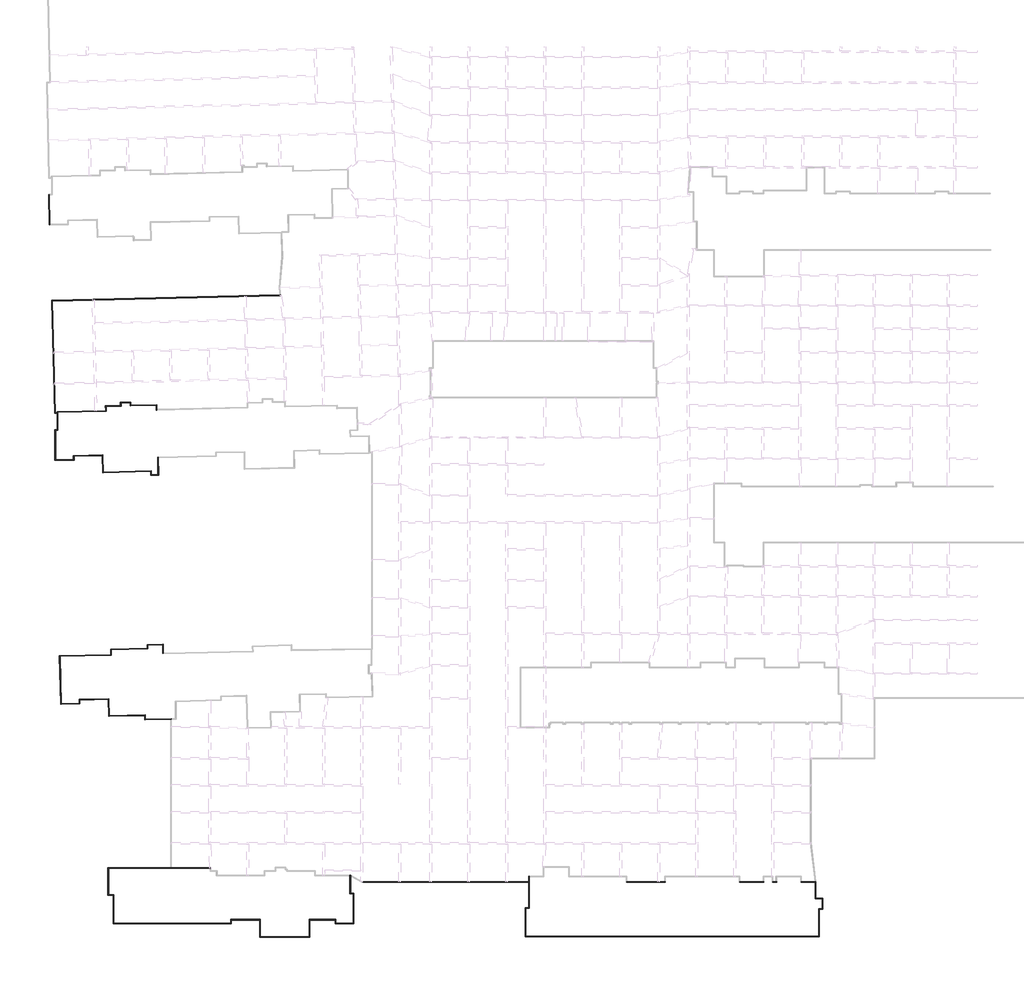
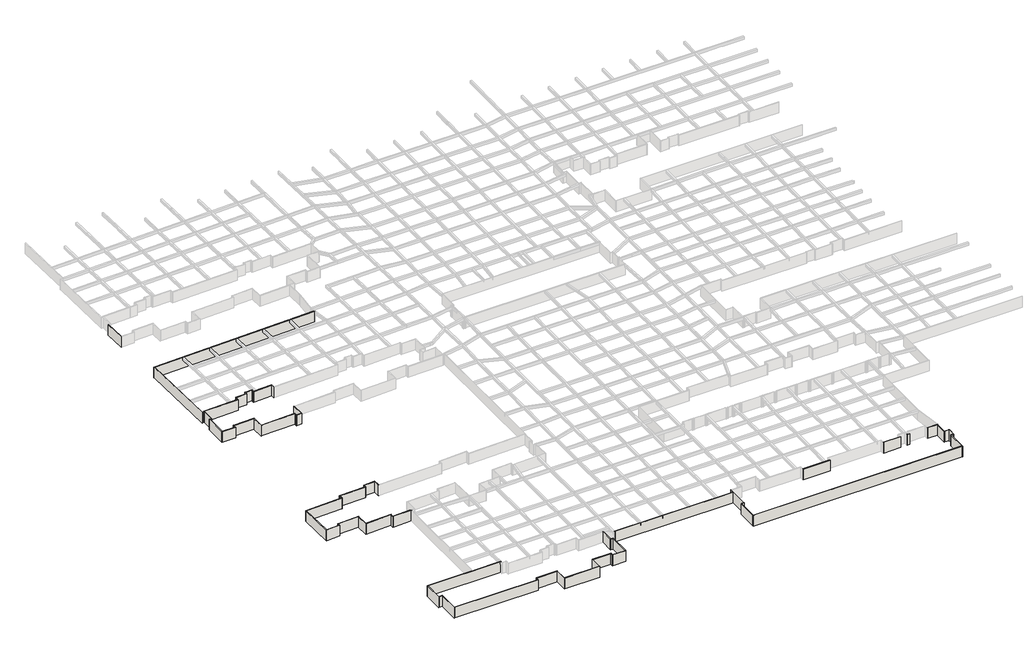
# One storey, part 1 of 20: 68 walls.
# Revit data of these elements (continued)
# Area, not placed, upper offset 0 mm, lower offset 0 mm (continued)
#   Number = "7"
#   Name = "fire_compart_5"
# Area, not placed, upper offset 0 mm, lower offset 0 mm
#   Number = "1"
#   Name = "面积"
# Area, not placed, upper offset 0 mm, lower offset 0 mm
#   Number = "2"
#   Name = "防火区域1"
# Area, not placed, upper offset 0 mm, lower offset 0 mm
#   Number = "25"
#   Name = "fire_compart"
# Area, not placed, upper offset 0 mm, lower offset 0 mm
#   Number = "26"
#   Name = "fire_compart"
# Area, not placed, upper offset 0 mm, lower offset 0 mm
#   Number = "27"
#   Name = "fire_compart"
# Room, not placed, phase "新构造", upper offset 0 mm, lower offset 0 mm
#   Number = "8"
#   Name = "客餐厅"
# Area, not placed, upper offset 0 mm, lower offset 0 mm
#   Number = "8"
#   Name = "fire_compart_6"
# Area, not placed, upper offset 0 mm, lower offset 0 mm
#   Number = "3"
#   Name = "fire_compart_1"
# Room, not placed, phase "新构造", upper offset 0 mm, lower offset 0 mm
#   Number = "11"
#   Name = "房间"
# Room, not placed, phase "新构造", upper offset 0 mm, lower offset 0 mm
#   Number = "12"
#   Name = "房间"
# Room, not placed, phase "新构造", upper offset 0 mm, lower offset 0 mm
#   Number = "13"
#   Name = "房间"
# Room, not placed, phase "新构造", upper offset 0 mm, lower offset 0 mm
#   Number = "14"
#   Name = "房间"
# Room, not placed, phase "新构造", upper offset 0 mm, lower offset 0 mm
#   Number = "15"
#   Name = "房间"
# Room, not placed, phase "新构造", upper offset 0 mm, lower offset 0 mm
#   Number = "16"
#   Name = "房间"
# Area, not placed, upper offset 0 mm, lower offset 0 mm
#   Number = "28"
#   Name = "面积"
# Room, not placed, phase "新构造", upper offset 0 mm, lower offset 0 mm
#   Number = "17"
#   Name = "房间"
# Area, not placed, upper offset 0 mm, lower offset 0 mm
#   Number = "30"
#   Name = "main_building"
# Area, not placed, upper offset 0 mm, lower offset 0 mm
#   Number = "4"
#   Name = "fire_compart_2"
# Area, not placed, upper offset 0 mm, lower offset 0 mm
#   Number = "29"
#   Name = "main_building"
